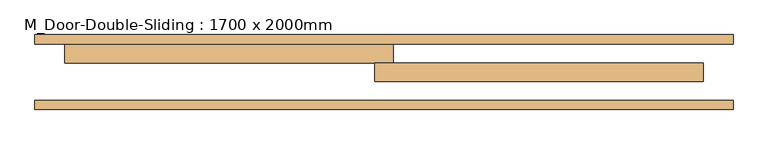
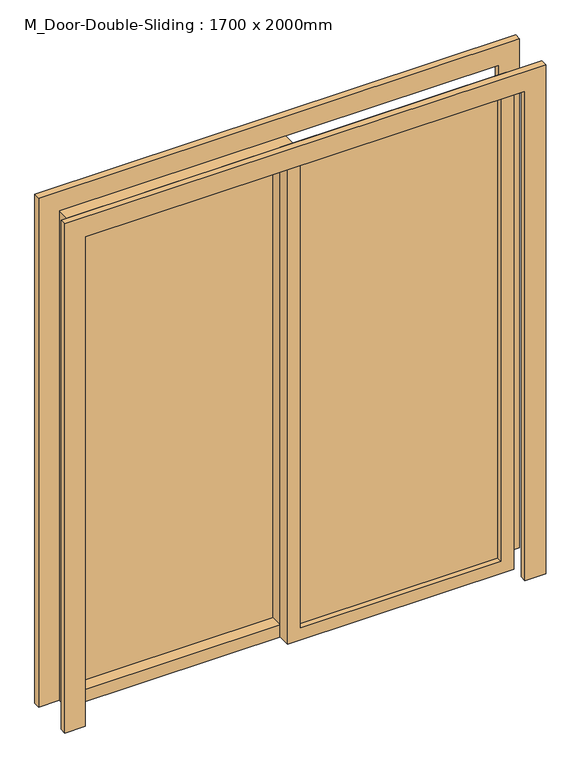
"""IFC4 building model written with IfcOpenShell, lengths in millimetres: door geometry, M_Door-Double-Sliding : 1700 x 2000mm."""

from ifc_helpers import new_model, si_unit, frame, origin, place, context, project, spatial, polyline, outline, extrude, source, transform, mapped, element, save


def m_door_double_sliding_1700_x_2000mm_d1f6b422(model_context):
    return source(origin(), model_context, "Body", "SweptSolid", [
        extrude(outline(polyline([(0.0, -930.0), (0.0, -850.0), (2000.0, -850.0), (2000.0, 850.0), (0.0, 850.0), (0.0, 930.0), (2080.0, 930.0), (2080.0, -930.0), (0.0, -930.0)])), frame((0.0, 27.0, 0.0), z_axis=(0.0, 1.0, 0.0), x_axis=(0.0, 0.0, 1.0)), (0.0, 0.0, 1.0), 25.0),
        extrude(outline(polyline([(0.0, 930.0), (2080.0, 930.0), (2080.0, -930.0), (0.0, -930.0), (0.0, -850.0), (2000.0, -850.0), (2000.0, 850.0), (0.0, 850.0), (0.0, 930.0)])), frame((0.0, 202.0, 0.0), z_axis=(0.0, 1.0, 0.0), x_axis=(0.0, 0.0, 1.0)), (0.0, 0.0, 1.0), 25.0),
        extrude(outline(polyline([(2000.0, -25.0), (0.0, -25.0), (0.0, 850.0), (2000.0, 850.0), (2000.0, -25.0)]), holes=[polyline([(1950.0, 25.0), (1950.0, 800.0), (50.0, 800.0), (50.0, 25.0), (1950.0, 25.0)])]), frame((0.0, 102.0, 0.0), z_axis=(0.0, 1.0, 0.0), x_axis=(0.0, 0.0, 1.0)), (0.0, 0.0, 1.0), 50.0),
        extrude(outline(polyline([(2000.0, 25.0), (2000.0, -850.0), (0.0, -850.0), (0.0, 25.0), (2000.0, 25.0)]), holes=[polyline([(1950.0, -25.0), (50.0, -25.0), (50.0, -800.0), (1950.0, -800.0), (1950.0, -25.0)])]), frame((0.0, 152.0, 0.0), z_axis=(0.0, 1.0, 0.0), x_axis=(0.0, 0.0, 1.0)), (0.0, 0.0, 1.0), 50.0),
        extrude(outline(polyline([(25.0, 130.175), (800.0, 130.175), (800.0, 123.825), (25.0, 123.825), (25.0, 130.175)])), frame((0.0, 0.0, 50.0), z_axis=(0.0, 0.0, 1.0), x_axis=(1.0, 0.0, 0.0)), (0.0, 0.0, 1.0), 1900.0),
        extrude(outline(polyline([(-25.0, 200.025), (-800.0, 200.025), (-800.0, 206.375), (-25.0, 206.375), (-25.0, 200.025)])), frame((0.0, 0.0, 50.0), z_axis=(0.0, 0.0, 1.0), x_axis=(1.0, 0.0, 0.0)), (0.0, 0.0, 1.0), 1900.0),
    ])


if __name__ == "__main__":
    model = new_model("IFC4")
    model_context = context("Model", 3, world=origin())
    ifc_project = project(units=[si_unit("LENGTHUNIT", "METRE", prefix="MILLI")], contexts=[model_context])
    site = spatial("IfcSite", under=ifc_project)
    building = spatial("IfcBuilding", under=site)
    placement = place(None, origin())
    m_door_double_sliding_1700_x_2000mm_shape = m_door_double_sliding_1700_x_2000mm_d1f6b422(model_context)
    element("IfcDoor", 1, ObjectType="M_Door-Double-Sliding : 1700 x 2000mm", at=placement, inside=building, context=model_context, shape_type="MappedRepresentation", body=[
        mapped(m_door_double_sliding_1700_x_2000mm_shape, transform((0.0, 0.0, 0.0), x_axis=(1.0, 0.0, 0.0), y_axis=(0.0, 1.0, 0.0), z_axis=(0.0, 0.0, 1.0))),
    ])
    save(model, "model.ifc")

# Revit data of these elements
# Type "M_Door-Double-Sliding : 1700 x 2000mm"
#   Type Mark = "22"
#   Construction Type Id = "opn-d45"
#   Assembly Code = "C1020"
#   Analytic Construction = "Wood frame, double glass door "
#   Thickness = 0.05 m
#   Thermal Resistance (R) = 0.31964 (m²·K)/W
#   Heat Transfer Coefficient (U) = 3.12872 W/(m²·K)
#   Height = 2 m
#   Rail Width = 0.05 m
#   Stiles = 0.05 m
#   Trim Projection Ext = 0.025 m
#   Trim Projection Int = 0.025 m
#   Trim Width = 0.08 m
#   Width = 1.7 m
#   Glazing = Glass
#   Panel Material = Wood - Birch - Solid Stained Light Low Gloss
#   Trim Material = Paint - Sienna
#   Visual Light Transmittance = 0
#   Solar Heat Gain Coefficient = 0
#   Function = (empty or 0)
#   Wall Closure = (empty or 0)
# Element 1 (IfcDoor, "M_Door-Double-Sliding : 1700 x 2000mm")
#   Materials on its faces: "Paint - Sienna", "Wood - Birch - Solid Stained Light Low Gloss", "Glass"
# Materials
#   "Glass": class "Glass", colour RGB 247 249 248, transparency 0.85, Description = "Soda Lime Glass", Cost = 0
#   "Wood - Birch - Solid Stained Light Low Gloss": class "Wood", colour RGB 227 170 128, transparency 0, Cost = 0
#   "Paint - Sienna": class "Miscellaneous", colour RGB 118 70 51, transparency 0, Cost = 0
